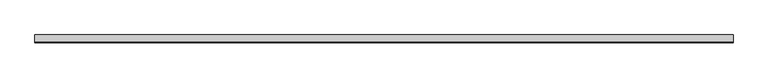
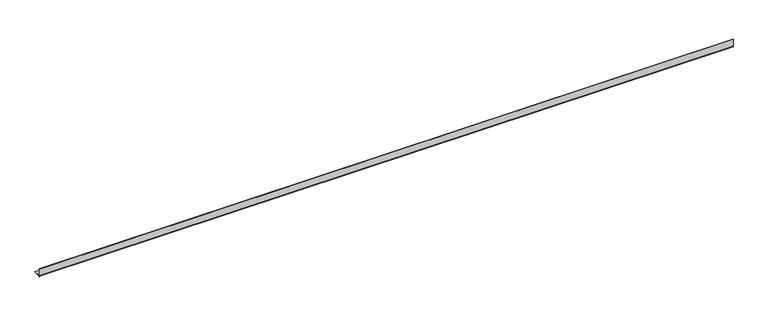
"""IFC4 building model written with IfcOpenShell, lengths in millimetres: proxy geometry, Metal profile001 197 : Metal profile001 197."""

from ifc_helpers import new_model, si_unit, point, frame, frame_2d, origin, place, context, project, spatial, polyline, circle_curve, trimmed, segment, composite_curve, outline, extrude, source, transform, mapped, element, save


def generic_models_db72ebd8(model_context):
    return source(origin(), model_context, "Body", "SweptSolid", [
        extrude(outline(composite_curve([segment(polyline([(10196.5677938, 39423.8851145), (10196.5677938, 39402.7319306), (10217.7209778, 39402.7319306), (10217.7209778, 39401.4519306), (10196.8180681, 39401.4519306)]), True, "CONTINUOUS"), segment(trimmed(circle_curve(frame_2d((10195.9277938, 39402.0919306)), 1.0964434), [point((10196.8180681, 39401.4519306))], [point((10195.2877938, 39402.9822048))], False, "CARTESIAN"), True, "CONTINUOUS"), segment(polyline([(10195.2877938, 39402.9822048), (10195.2877938, 39423.8851145), (10196.5677938, 39423.8851145)]), True, "CONTINUOUS")], self_intersect=False)), frame((3694.2883192, 0.0, 0.0), z_axis=(1.0, 0.0, 0.0), x_axis=(0.0, 1.0, 0.0)), (0.0, 0.0, 1.0), 2000.0),
    ])


if __name__ == "__main__":
    model = new_model("IFC4")
    model_context = context("Model", 3, world=origin())
    ifc_project = project(units=[si_unit("LENGTHUNIT", "METRE", prefix="MILLI")], contexts=[model_context])
    site = spatial("IfcSite", under=ifc_project)
    building = spatial("IfcBuilding", under=site)
    placement = place(None, origin())
    generic_models_shape = generic_models_db72ebd8(model_context)
    element("IfcBuildingElementProxy", 1, Name="Metal profile001 197 : Metal profile001 197", ObjectType="Metal profile001 197 : Metal profile001 197", at=placement, inside=building, context=model_context, shape_type="MappedRepresentation", body=[
        mapped(generic_models_shape, transform((0.0, 0.0, 0.0), x_axis=(1.0, 0.0, 0.0), y_axis=(0.0, 1.0, 0.0), z_axis=(0.0, 0.0, 1.0))),
    ])
    save(model, "model.ifc")

# Revit data of these elements
# Type "Metal profile001 197 : Metal profile001 197"
#   NameOverride = "Metal profile001"
# Element 1 (IfcBuildingElementProxy, "Metal profile001 197 : Metal profile001 197")
#   Materials on its faces: "CORNER BEAD"
# Materials
#   "CORNER BEAD": class "Unassigned", colour RGB 255 241 0, transparency 0
